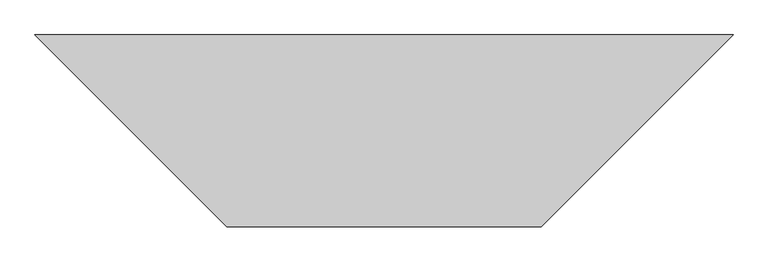
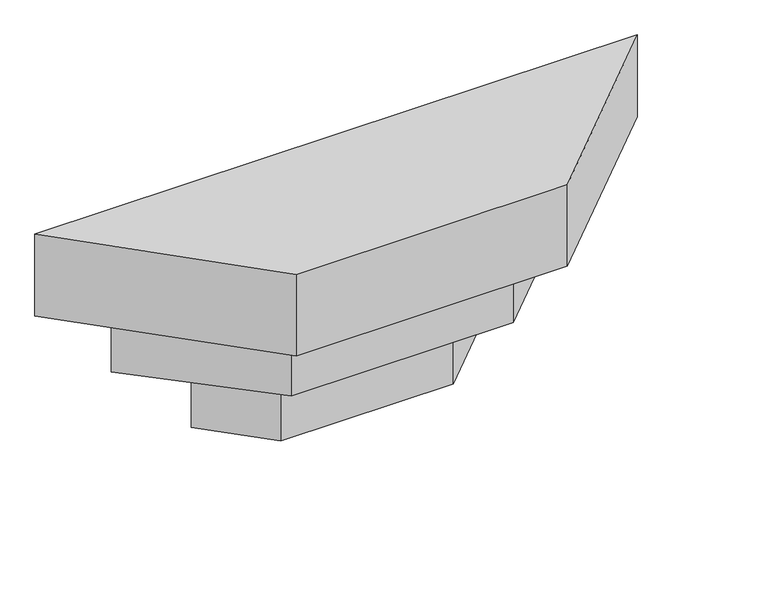
"""IFC4 building model written with IfcOpenShell, lengths in millimetres: furniture geometry, Bay Window fake support : Bay Window fake support."""

from ifc_helpers import new_model, si_unit, frame, origin, place, context, project, spatial, polyline, outline, extrude, source, transform, mapped, element, save


def furniture_e9cff47f(model_context):
    return source(origin(), model_context, "Body", "SweptSolid", [
        extrude(outline(polyline([(6997.8279394, 5715.5894472), (6315.3284742, 5033.089982), (5197.7284742, 5033.089982), (4515.229009, 5715.5894472), (6997.8279394, 5715.5894472)])), frame((0.0, 0.0, -965.2), z_axis=(0.0, 0.0, 1.0), x_axis=(1.0, 0.0, 0.0)), (0.0, 0.0, 1.0), 355.6),
        extrude(outline(polyline([(6675.0101826, 5715.5894472), (6225.9973766, 5266.5766411), (5311.5973766, 5266.5766411), (4830.090093, 5715.5894472), (6675.0101826, 5715.5894472)])), frame((0.0, 0.0, -1320.8), z_axis=(0.0, 0.0, 1.0), x_axis=(1.0, 0.0, 0.0)), (0.0, 0.0, 1.0), 355.6),
        extrude(outline(polyline([(6338.1943864, 5715.2944638), (6104.7077273, 5481.8078047), (5393.5077273, 5481.8078047), (5160.0210681, 5715.2944638), (6338.1943864, 5715.2944638)])), frame((0.0, 0.0, -1676.4), z_axis=(0.0, 0.0, 1.0), x_axis=(1.0, 0.0, 0.0)), (0.0, 0.0, 1.0), 355.6),
    ])


if __name__ == "__main__":
    model = new_model("IFC4")
    model_context = context("Model", 3, world=origin())
    ifc_project = project(units=[si_unit("LENGTHUNIT", "METRE", prefix="MILLI")], contexts=[model_context])
    site = spatial("IfcSite", under=ifc_project)
    building = spatial("IfcBuilding", under=site)
    placement = place(None, origin())
    furniture_shape = furniture_e9cff47f(model_context)
    element("IfcFurniture", 1, ObjectType="Bay Window fake support : Bay Window fake support", at=placement, inside=building, context=model_context, shape_type="MappedRepresentation", body=[
        mapped(furniture_shape, transform((0.0, 0.0, 0.0), x_axis=(1.0, 0.0, 0.0), y_axis=(0.0, 1.0, 0.0), z_axis=(0.0, 0.0, 1.0))),
    ])
    save(model, "model.ifc")

# Revit data of these elements
# Type "Bay Window fake support : Bay Window fake support"
#   COBie.Type = no
# Element 1 (IfcFurniture, "Bay Window fake support : Bay Window fake support")
#   Materials on its faces: "Trim - White"
# Materials
#   "Trim - White": class "Wood", colour RGB 255 255 255, transparency 0, Cost = 0
